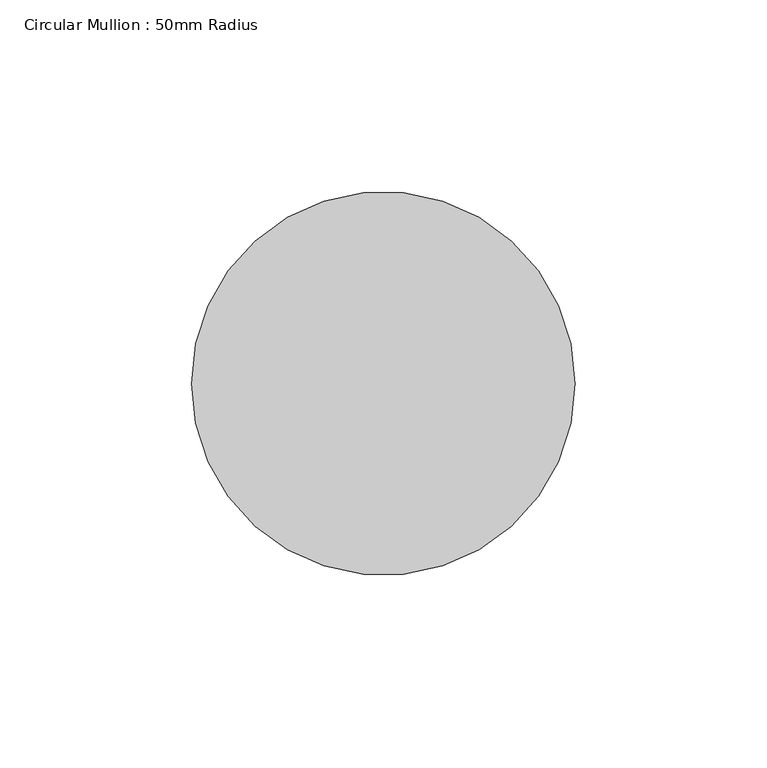
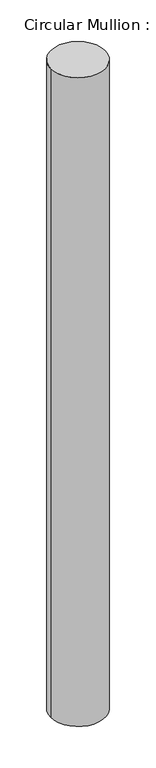
"""IFC4 building model written with IfcOpenShell, lengths in millimetres: member geometry, Circular Mullion : 50mm Radius."""

from ifc_helpers import new_model, si_unit, point, frame, origin, origin_2d, place, context, project, spatial, circle_curve, trimmed, segment, composite_curve, outline, extrude, source, transform, mapped, element, save


def circular_mullion_50mm_radius_5a809ce4(model_context):
    return source(origin(), model_context, "Body", "SweptSolid", [
        extrude(outline(composite_curve([segment(trimmed(circle_curve(origin_2d(), 50.0), [point((50.0, 0.0))], [point((-50.0, 0.0))], False, "CARTESIAN"), True, "CONTINUOUS"), segment(trimmed(circle_curve(origin_2d(), 50.0), [point((-50.0, 0.0))], [point((50.0, 0.0))], False, "CARTESIAN"), True, "CONTINUOUS")], self_intersect=False)), frame((0.0, 0.0, -1257.1978721), z_axis=(0.0, 0.0, 1.0), x_axis=(1.0, 0.0, 0.0)), (0.0, 0.0, 1.0), 1257.1978721),
    ])


if __name__ == "__main__":
    model = new_model("IFC4")
    model_context = context("Model", 3, world=origin())
    ifc_project = project(units=[si_unit("LENGTHUNIT", "METRE", prefix="MILLI")], contexts=[model_context])
    site = spatial("IfcSite", under=ifc_project)
    building = spatial("IfcBuilding", under=site)
    placement = place(None, origin())
    circular_mullion_50mm_radius_shape = circular_mullion_50mm_radius_5a809ce4(model_context)
    element("IfcMember", 1, ObjectType="Circular Mullion : 50mm Radius", at=placement, inside=building, context=model_context, shape_type="MappedRepresentation", body=[
        mapped(circular_mullion_50mm_radius_shape, transform((0.0, 0.0, 0.0), x_axis=(1.0, 0.0, 0.0), y_axis=(0.0, 1.0, 0.0), z_axis=(0.0, 0.0, 1.0))),
    ])
    save(model, "model.ifc")

# Revit data of these elements
# Type "Circular Mullion : 50mm Radius"
#   built-in parameter 1007350 = 0.164042 (stored number, unit not read)
# Element 1 (IfcMember, "Circular Mullion : 50mm Radius")
#   Materials on its faces: "Aluminium"
# Materials
#   "Aluminium": class "Metal", colour RGB 247 247 247, transparency 0, Description = "Aluminium 6061", Cost = 0
